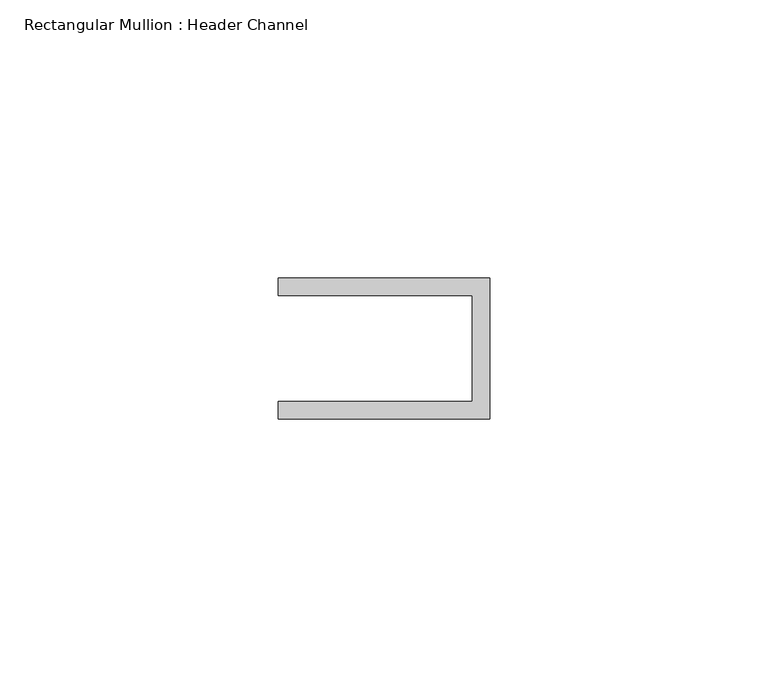
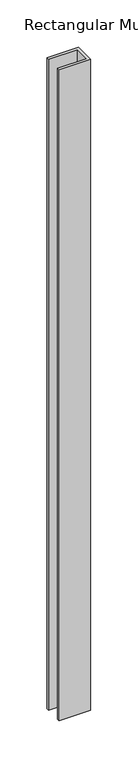
"""IFC4 building model written with IfcOpenShell, lengths in millimetres: member geometry, Rectangular Mullion : Header Channel."""

from ifc_helpers import new_model, si_unit, frame, origin, place, context, project, spatial, polyline, outline, extrude, source, transform, mapped, element, save


def rectangular_mullion_header_channel_0f02b38c(model_context):
    return source(origin(), model_context, "Body", "SweptSolid", [
        extrude(outline(polyline([(0.0, -12.7), (-38.1, -12.7), (-38.1, -9.525), (-3.175, -9.525), (-3.175, 9.525), (-38.1, 9.525), (-38.1, 12.7), (0.0, 12.7), (0.0, -12.7)])), frame((0.0, 0.0, -838.1999999), z_axis=(0.0, 0.0, 1.0), x_axis=(1.0, 0.0, 0.0)), (0.0, 0.0, 1.0), 838.1999999),
    ])


if __name__ == "__main__":
    model = new_model("IFC4")
    model_context = context("Model", 3, world=origin())
    ifc_project = project(units=[si_unit("LENGTHUNIT", "METRE", prefix="MILLI")], contexts=[model_context])
    site = spatial("IfcSite", under=ifc_project)
    building = spatial("IfcBuilding", under=site)
    placement = place(None, origin())
    rectangular_mullion_header_channel_shape = rectangular_mullion_header_channel_0f02b38c(model_context)
    element("IfcMember", 1, ObjectType="Rectangular Mullion : Header Channel", at=placement, inside=building, context=model_context, shape_type="MappedRepresentation", body=[
        mapped(rectangular_mullion_header_channel_shape, transform((0.0, 0.0, 0.0), x_axis=(1.0, 0.0, 0.0), y_axis=(0.0, 1.0, 0.0), z_axis=(0.0, 0.0, 1.0))),
    ])
    save(model, "model.ifc")

# Revit data of these elements
# Type "Rectangular Mullion : Header Channel"
#   built-in parameter 1007322 = 0.0833333 (stored number, unit not read)
#   built-in parameter 1007321 = -0.03125 (stored number, unit not read)
#   built-in parameter 1007320 = 0.0416667 (stored number, unit not read)
# Element 1 (IfcMember, "Rectangular Mullion : Header Channel")
#   Materials on its faces: "ALUM"
# Materials
#   "ALUM": class "Generic", colour RGB 157 157 157, transparency 0, Cost = 0
